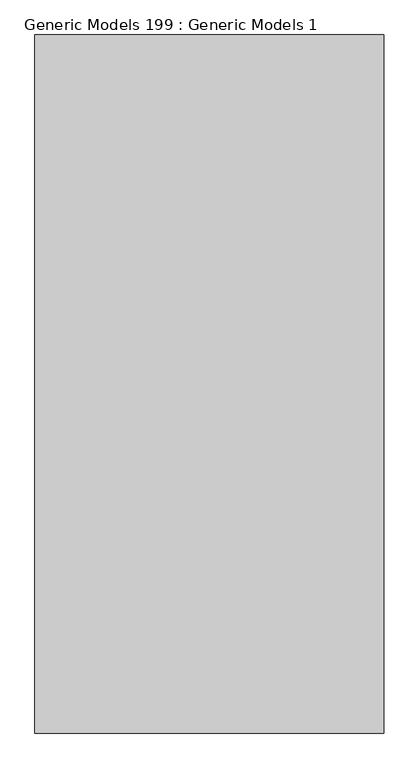
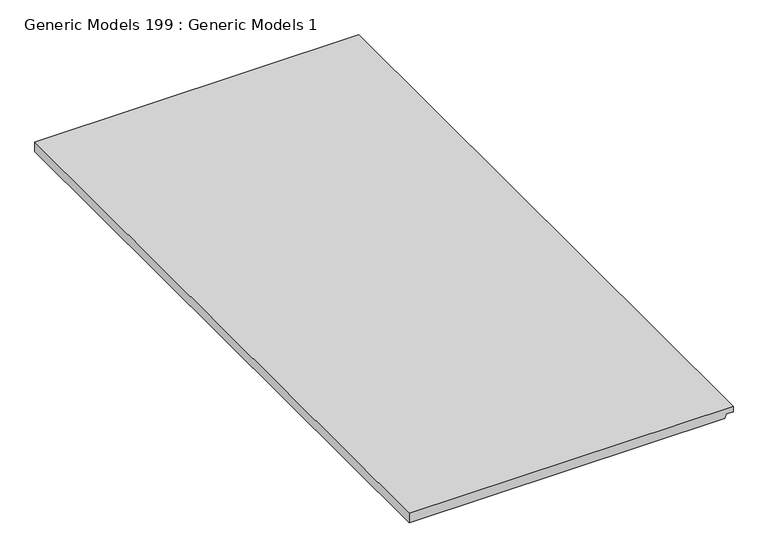
"""IFC4 building model written with IfcOpenShell, lengths in millimetres: proxy geometry, Generic Models 199 : Generic Models 1."""

from ifc_helpers import new_model, si_unit, frame, origin, place, context, project, spatial, polyline, outline, extrude, source, transform, mapped, element, save


def generic_models_199_generic_models_1_28f40251(model_context):
    return source(origin(), model_context, "Body", "SweptSolid", [
        extrude(outline(polyline([(2253.330428, 49662.5798593), (2253.330428, 49052.9798593), (2234.280428, 49052.9798593), (2234.280428, 49646.9908455), (2242.217928, 49649.8798593), (2242.217928, 49662.5798593), (2253.330428, 49662.5798593)])), frame((0.0, 0.0, 0.0), z_axis=(0.0, 1.0, 0.0), x_axis=(0.0, 0.0, 1.0)), (0.0, 0.0, 1.0), 1219.2),
    ])


if __name__ == "__main__":
    model = new_model("IFC4")
    model_context = context("Model", 3, world=origin())
    ifc_project = project(units=[si_unit("LENGTHUNIT", "METRE", prefix="MILLI")], contexts=[model_context])
    site = spatial("IfcSite", under=ifc_project)
    building = spatial("IfcBuilding", under=site)
    placement = place(None, origin())
    generic_models_199_generic_models_1_shape = generic_models_199_generic_models_1_28f40251(model_context)
    element("IfcBuildingElementProxy", 1, Name="Generic Models 199 : Generic Models 1", ObjectType="Generic Models 199 : Generic Models 1", at=placement, inside=building, context=model_context, shape_type="MappedRepresentation", body=[
        mapped(generic_models_199_generic_models_1_shape, transform((0.0, 0.0, 0.0), x_axis=(1.0, 0.0, 0.0), y_axis=(0.0, 1.0, 0.0), z_axis=(0.0, 0.0, 1.0))),
    ])
    save(model, "model.ifc")

# Revit data of these elements
# Element 1 (IfcBuildingElementProxy, "Generic Models 199 : Generic Models 1")
#   Materials on its faces: "CEILING AS SCHEDULED"
# Materials
#   "CEILING AS SCHEDULED": class "Generic", colour RGB 255 255 255, transparency 0, Cost = 0
